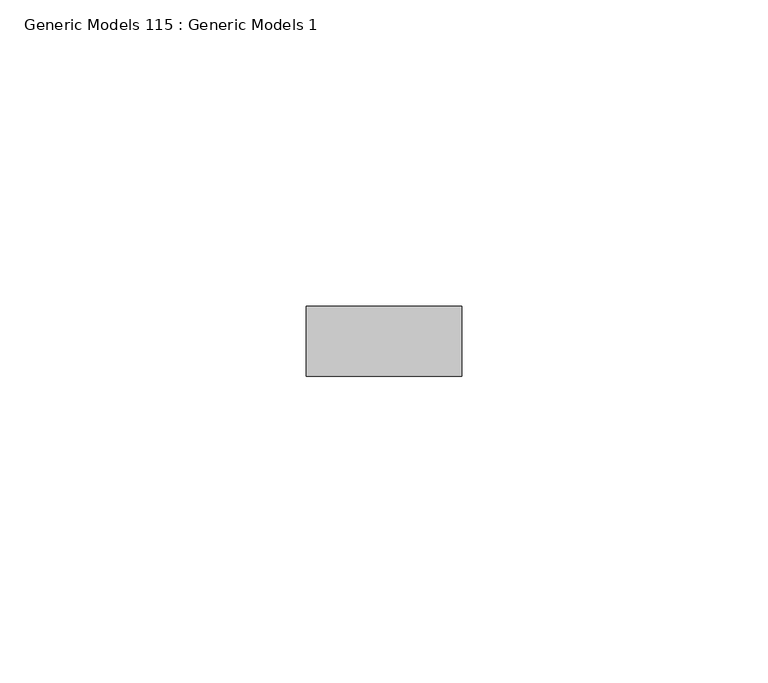
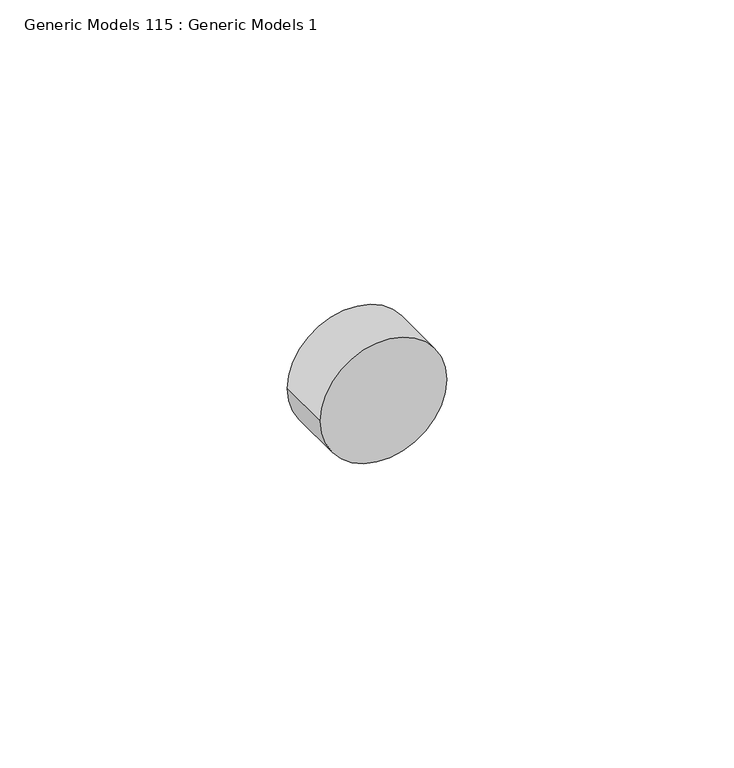
"""IFC4 building model written with IfcOpenShell, lengths in millimetres: proxy geometry, Generic Models 115 : Generic Models 1."""

from ifc_helpers import new_model, si_unit, point, frame, frame_2d, origin, place, context, project, spatial, circle_curve, trimmed, segment, composite_curve, outline, extrude, source, transform, mapped, element, save


def generic_models_115_generic_models_1_a7f3b69d(model_context):
    return source(origin(), model_context, "Body", "SweptSolid", [
        extrude(outline(composite_curve([segment(trimmed(circle_curve(frame_2d((37860.4162436, 6738.7346014)), 12.7), [point((37860.4162436, 6751.4346014))], [point((37860.4162436, 6726.0346014))], False, "CARTESIAN"), True, "CONTINUOUS"), segment(trimmed(circle_curve(frame_2d((37860.4162436, 6738.7346014)), 12.7), [point((37860.4162436, 6726.0346014))], [point((37860.4162436, 6751.4346014))], False, "CARTESIAN"), True, "CONTINUOUS")], self_intersect=False)), frame((0.0, 1836.9202358, 0.0), z_axis=(0.0, 1.0, 0.0), x_axis=(0.0, 0.0, 1.0)), (0.0, 0.0, 1.0), 11.4464372),
    ])


if __name__ == "__main__":
    model = new_model("IFC4")
    model_context = context("Model", 3, world=origin())
    ifc_project = project(units=[si_unit("LENGTHUNIT", "METRE", prefix="MILLI")], contexts=[model_context])
    site = spatial("IfcSite", under=ifc_project)
    building = spatial("IfcBuilding", under=site)
    placement = place(None, origin())
    generic_models_115_generic_models_1_shape = generic_models_115_generic_models_1_a7f3b69d(model_context)
    element("IfcBuildingElementProxy", 1, Name="Generic Models 115 : Generic Models 1", ObjectType="Generic Models 115 : Generic Models 1", at=placement, inside=building, context=model_context, shape_type="MappedRepresentation", body=[
        mapped(generic_models_115_generic_models_1_shape, transform((0.0, 0.0, 0.0), x_axis=(1.0, 0.0, 0.0), y_axis=(0.0, 1.0, 0.0), z_axis=(0.0, 0.0, 1.0))),
    ])
    save(model, "model.ifc")

# Revit data of these elements
# Element 1 (IfcBuildingElementProxy, "Generic Models 115 : Generic Models 1")
#   Materials on its faces: "S.S. LAG BOLT - SEE STRUCT. DWGS"
# Materials
#   "S.S. LAG BOLT - SEE STRUCT. DWGS": class "Generic", colour RGB 120 120 120, transparency 0, Cost = 0
